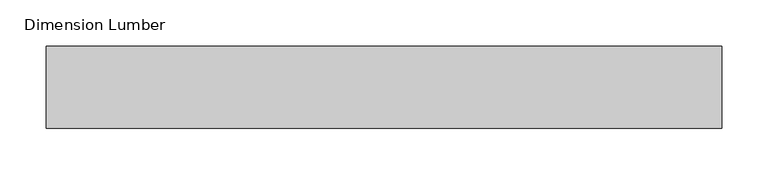
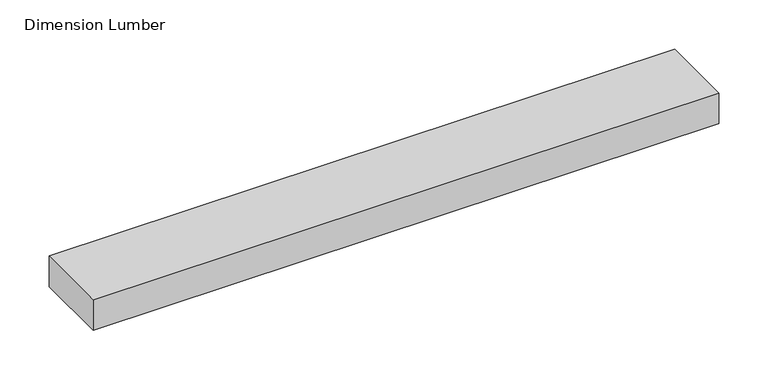
"""IFC4 building model written with IfcOpenShell, lengths in millimetres: beam geometry, Dimension Lumber : Top Supporting Lumbers."""

from ifc_helpers import new_model, si_unit, frame, origin, place, context, project, spatial, polyline, outline, extrude, source, transform, mapped, element, save


def dimension_lumber_74193215(model_context):
    return source(origin(), model_context, "Body", "SweptSolid", [
        extrude(outline(polyline([(409.575, 44.45), (409.575, -44.45), (-320.675, -44.45), (-320.675, 44.45), (409.575, 44.45)])), frame((0.0, 0.0, -19.05), z_axis=(0.0, 0.0, 1.0), x_axis=(1.0, 0.0, 0.0)), (0.0, 0.0, 1.0), 38.1),
    ])


if __name__ == "__main__":
    model = new_model("IFC4")
    model_context = context("Model", 3, world=origin())
    ifc_project = project(units=[si_unit("LENGTHUNIT", "METRE", prefix="MILLI")], contexts=[model_context])
    site = spatial("IfcSite", under=ifc_project)
    building = spatial("IfcBuilding", under=site)
    placement = place(None, origin())
    dimension_lumber_shape = dimension_lumber_74193215(model_context)
    element("IfcBeam", 1, ObjectType="Dimension Lumber : Top Supporting Lumbers", at=placement, inside=building, context=model_context, shape_type="MappedRepresentation", body=[
        mapped(dimension_lumber_shape, transform((0.0, 0.0, 0.0), x_axis=(1.0, 0.0, 0.0), y_axis=(0.0, 1.0, 0.0), z_axis=(0.0, 0.0, 1.0))),
    ])
    save(model, "model.ifc")

# Revit data of these elements
# Type "Dimension Lumber : Top Supporting Lumbers"
#   Assembly Code = "B10"
#   A = 0.0364583 SF
#   Length [instance default] = 5' - 0"
#   b = 0' - 3 1/2"
#   d = 0' - 1 1/2"
#   Structural Material [instance default] = Softwood, Lumber
# Element 1 (IfcBeam, "Dimension Lumber : Top Supporting Lumbers")
#   Structural Material = Douglas Fir #2
#   Materials on its faces: "Douglas Fir #2"
# Materials
#   "Softwood, Lumber": class "Wood", colour RGB 223 192 134, transparency 0, Description = "Pinus Echinata", Cost = 0
#   "Douglas Fir #2": class "Wood", colour RGB 223 192 134, transparency 0, Description = "Pinus Echinata", Cost = 0
